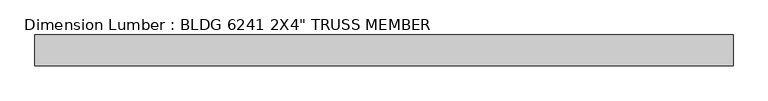
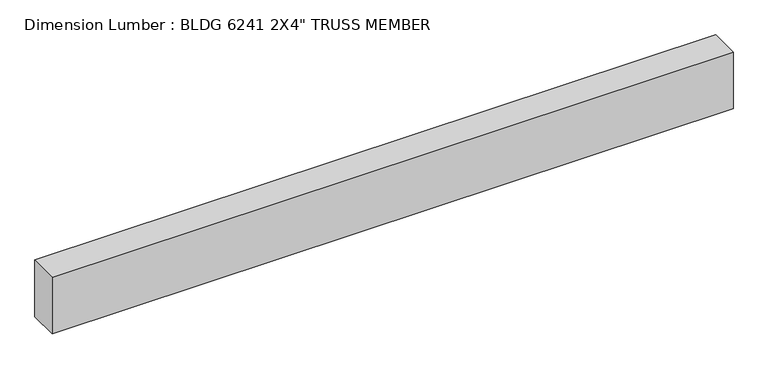
"""IFC4 building model written with IfcOpenShell, lengths in millimetres: beam geometry."""

from ifc_helpers import new_model, si_unit, frame, origin, place, context, project, spatial, polyline, outline, extrude, source, transform, mapped, element, save


def beam_f5027b49(model_context):
    return source(origin(), model_context, "Body", "SweptSolid", [
        extrude(outline(polyline([(571.5, 25.4), (571.5, -25.4), (-584.2, -25.4), (-584.2, 25.4), (571.5, 25.4)])), frame((0.0, 0.0, -50.8), z_axis=(0.0, 0.0, 1.0), x_axis=(1.0, 0.0, 0.0)), (0.0, 0.0, 1.0), 101.6),
    ])


if __name__ == "__main__":
    model = new_model("IFC4")
    model_context = context("Model", 3, world=origin())
    ifc_project = project(units=[si_unit("LENGTHUNIT", "METRE", prefix="MILLI")], contexts=[model_context])
    site = spatial("IfcSite", under=ifc_project)
    building = spatial("IfcBuilding", under=site)
    placement = place(None, origin())
    beam_shape = beam_f5027b49(model_context)
    element("IfcBeam", 1, ObjectType="Dimension Lumber : BLDG 6241 2X4\" TRUSS MEMBER", at=placement, inside=building, context=model_context, shape_type="MappedRepresentation", body=[
        mapped(beam_shape, transform((0.0, 0.0, 0.0), x_axis=(1.0, 0.0, 0.0), y_axis=(0.0, 1.0, 0.0), z_axis=(0.0, 0.0, 1.0))),
    ])
    save(model, "model.ifc")

# Revit data of these elements
# Type "Dimension Lumber : BLDG 6241 2X4\" TRUSS MEMBER"
#   Assembly Code = "B10"
#   A = 0.273472 SF
#   Length [instance default] = 5' - 0"
#   b = 0' - 2"
#   d = 0' - 4"
#   Structural Material [instance default] = Softwood, Lumber
# Element 1 (IfcBeam, "Dimension Lumber : BLDG 6241 2X4\" TRUSS MEMBER")
#   Materials on its faces: "Softwood, Lumber"
# Materials
#   "Softwood, Lumber": class "Wood", colour RGB 223 192 134, transparency 0, Description = "Pinus Echinata", Cost = 0
